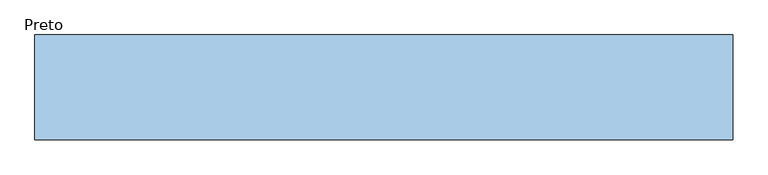
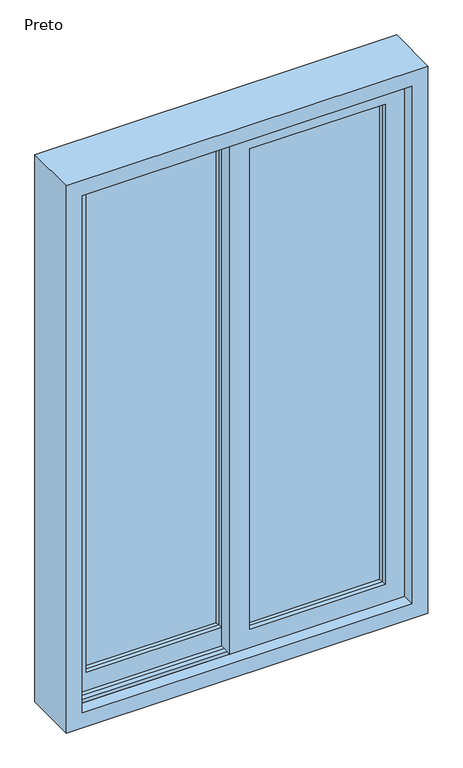
"""IFC4 building model written with IfcOpenShell, lengths in millimetres: window geometry, Blks_Cons Weiku_Janela de Correr 02 Folhas : Preto."""

from ifc_helpers import new_model, si_unit, frame, origin, place, context, project, spatial, polyline, outline, extrude, faceted_brep, source, transform, mapped, element, save


def preto_50c638ee(model_context):
    return source(origin(), model_context, "Body", "SolidModel", [
        faceted_brep([(27.0, -13.0, 898.0), (27.0, -18.0, 898.0), (27.0, -18.0, 2302.0), (27.0, -13.0, 2302.0), (32.0, -18.0, 903.0), (32.0, -18.0, 2297.0), (402.0, -18.0, 2302.0), (402.0, -13.0, 2302.0), (397.0, -18.0, 2297.0), (402.0, -18.0, 898.0), (402.0, -13.0, 898.0), (397.0, -18.0, 903.0)], [[[0, 1, 2, 3]], [[4, 0, 3, 5]], [[3, 2, 6, 7]], [[5, 3, 7, 8]], [[7, 6, 9, 10]], [[8, 7, 10, 11]], [[1, 9, 6, 2], [5, 8, 11, 4]], [[10, 9, 1, 0]], [[11, 10, 0, 4]]]),
        faceted_brep([(402.0, -27.0, 898.0), (402.0, -22.0, 898.0), (402.0, -22.0, 2302.0), (402.0, -27.0, 2302.0), (27.0, -22.0, 2302.0), (27.0, -27.0, 2302.0), (27.0, -22.0, 898.0), (27.0, -27.0, 898.0), (397.0, -22.0, 2297.0), (32.0, -22.0, 2297.0), (32.0, -22.0, 903.0), (397.0, -22.0, 903.0)], [[[0, 1, 2, 3]], [[3, 2, 4, 5]], [[5, 4, 6, 7]], [[1, 6, 4, 2], [8, 9, 10, 11]], [[7, 6, 1, 0]], [[11, 0, 3, 8]], [[8, 3, 5, 9]], [[9, 5, 7, 10]], [[10, 7, 0, 11]]]),
        extrude(outline(polyline([(402.0, -22.0), (27.0, -22.0), (27.0, -18.0), (402.0, -18.0), (402.0, -22.0)])), frame((0.0, 0.0, 898.0), z_axis=(0.0, 0.0, 1.0), x_axis=(1.0, 0.0, 0.0)), (0.0, 0.0, 1.0), 1404.0),
        extrude(outline(polyline([(844.0, 456.0), (2356.0, 456.0), (2356.0, -27.0), (844.0, -27.0), (844.0, 456.0)]), holes=[polyline([(2302.0, 27.0), (2302.0, 402.0), (898.0, 402.0), (898.0, 27.0), (2302.0, 27.0)])]), frame((0.0, -40.0, 0.0), z_axis=(0.0, 1.0, 0.0), x_axis=(0.0, 0.0, 1.0)), (0.0, 0.0, 1.0), 40.0),
        faceted_brep([(-402.0, 27.0, 898.0), (-402.0, 22.0, 898.0), (-402.0, 22.0, 2302.0), (-402.0, 27.0, 2302.0), (-397.0, 22.0, 903.0), (-397.0, 22.0, 2297.0), (-27.0, 22.0, 2302.0), (-27.0, 27.0, 2302.0), (-32.0, 22.0, 2297.0), (-27.0, 22.0, 898.0), (-27.0, 27.0, 898.0), (-32.0, 22.0, 903.0)], [[[0, 1, 2, 3]], [[4, 0, 3, 5]], [[3, 2, 6, 7]], [[5, 3, 7, 8]], [[7, 6, 9, 10]], [[8, 7, 10, 11]], [[1, 9, 6, 2], [5, 8, 11, 4]], [[10, 9, 1, 0]], [[11, 10, 0, 4]]]),
        faceted_brep([(-27.0, 13.0, 898.0), (-27.0, 18.0, 898.0), (-27.0, 18.0, 2302.0), (-27.0, 13.0, 2302.0), (-402.0, 18.0, 2302.0), (-402.0, 13.0, 2302.0), (-402.0, 18.0, 898.0), (-402.0, 13.0, 898.0), (-32.0, 18.0, 2297.0), (-397.0, 18.0, 2297.0), (-397.0, 18.0, 903.0), (-32.0, 18.0, 903.0)], [[[0, 1, 2, 3]], [[3, 2, 4, 5]], [[5, 4, 6, 7]], [[1, 6, 4, 2], [8, 9, 10, 11]], [[7, 6, 1, 0]], [[11, 0, 3, 8]], [[8, 3, 5, 9]], [[9, 5, 7, 10]], [[10, 7, 0, 11]]]),
        extrude(outline(polyline([(-27.0, 18.0), (-402.0, 18.0), (-402.0, 22.0), (-27.0, 22.0), (-27.0, 18.0)])), frame((0.0, 0.0, 898.0), z_axis=(0.0, 0.0, 1.0), x_axis=(1.0, 0.0, 0.0)), (0.0, 0.0, 1.0), 1404.0),
        extrude(outline(polyline([(844.0, 27.0), (2356.0, 27.0), (2356.0, -456.0), (844.0, -456.0), (844.0, 27.0)]), holes=[polyline([(2302.0, -402.0), (2302.0, -27.0), (898.0, -27.0), (898.0, -402.0), (2302.0, -402.0)])]), frame((0.0, 0.0, 0.0), z_axis=(0.0, 1.0, 0.0), x_axis=(0.0, 0.0, 1.0)), (0.0, 0.0, 1.0), 40.0),
        faceted_brep([(456.0, 75.0, 844.0), (-456.0, 75.0, 844.0), (-456.0, 40.0, 844.0), (456.0, 40.0, 844.0), (-456.0, -75.0, 844.0), (456.0, -75.0, 844.0), (456.0, -40.0, 844.0), (-456.0, -40.0, 844.0), (-456.0, -13.0, 844.0), (-456.0, -27.0, 844.0), (456.0, -27.0, 844.0), (456.0, -13.0, 844.0), (-456.0, 27.0, 844.0), (-456.0, 13.0, 844.0), (456.0, 13.0, 844.0), (456.0, 27.0, 844.0), (500.0, 75.0, 800.0), (-500.0, 75.0, 800.0), (-500.0, 75.0, 2400.0), (500.0, 75.0, 2400.0), (456.0, 75.0, 2356.0), (-456.0, 75.0, 2356.0), (-456.0, 40.0, 2356.0), (-456.0, 40.0, 2366.0), (-456.0, 27.0, 2366.0), (-456.0, 27.0, 2356.0), (-456.0, 13.0, 2356.0), (-456.0, 13.0, 2366.0), (-456.0, -13.0, 2366.0), (-456.0, -13.0, 2356.0), (-456.0, -27.0, 2356.0), (-456.0, -27.0, 2366.0), (-456.0, -40.0, 2366.0), (-456.0, -40.0, 2356.0), (-456.0, -75.0, 2356.0), (-456.0, -40.0, 834.0), (-456.0, -27.0, 834.0), (-456.0, -13.0, 834.0), (-456.0, 13.0, 834.0), (-456.0, 27.0, 834.0), (-456.0, 40.0, 834.0), (456.0, 40.0, 834.0), (456.0, 27.0, 834.0), (456.0, 13.0, 834.0), (456.0, -13.0, 834.0), (456.0, -27.0, 834.0), (456.0, -40.0, 834.0), (456.0, -75.0, 2356.0), (456.0, -40.0, 2356.0), (456.0, -40.0, 2366.0), (456.0, -27.0, 2366.0), (456.0, -27.0, 2356.0), (456.0, -13.0, 2356.0), (456.0, -13.0, 2366.0), (456.0, 13.0, 2366.0), (456.0, 13.0, 2356.0), (456.0, 27.0, 2356.0), (456.0, 27.0, 2366.0), (456.0, 40.0, 2366.0), (456.0, 40.0, 2356.0), (-500.0, -75.0, 800.0), (500.0, -75.0, 800.0), (500.0, -75.0, 2400.0), (-500.0, -75.0, 2400.0)], [[[0, 1, 2, 3]], [[4, 5, 6, 7]], [[8, 9, 10, 11]], [[12, 13, 14, 15]], [[16, 17, 18, 19], [1, 0, 20, 21]], [[1, 21, 22, 23, 24, 25, 26, 27, 28, 29, 30, 31, 32, 33, 34, 4, 7, 35, 36, 9, 8, 37, 38, 13, 12, 39, 40, 2]], [[40, 41, 3, 2]], [[20, 0, 3, 41, 42, 15, 14, 43, 44, 11, 10, 45, 46, 6, 5, 47, 48, 49, 50, 51, 52, 53, 54, 55, 56, 57, 58, 59]], [[60, 61, 62, 63], [5, 4, 34, 47]], [[46, 35, 7, 6]], [[45, 10, 9, 36]], [[11, 44, 37, 8]], [[43, 14, 13, 38]], [[15, 42, 39, 12]], [[61, 16, 19, 62]], [[16, 61, 60, 17]], [[17, 60, 63, 18]], [[46, 45, 36, 35]], [[44, 43, 38, 37]], [[42, 41, 40, 39]], [[26, 25, 56, 55]], [[30, 29, 52, 51]], [[21, 20, 59, 22]], [[47, 34, 33, 48]], [[18, 63, 62, 19]], [[55, 54, 27, 26]], [[54, 53, 28, 27]], [[53, 52, 29, 28]], [[51, 50, 31, 30]], [[50, 49, 32, 31]], [[32, 49, 48, 33]], [[58, 23, 22, 59]], [[58, 57, 24, 23]], [[57, 56, 25, 24]]]),
    ])


if __name__ == "__main__":
    model = new_model("IFC4")
    model_context = context("Model", 3, world=origin())
    ifc_project = project(units=[si_unit("LENGTHUNIT", "METRE", prefix="MILLI")], contexts=[model_context])
    site = spatial("IfcSite", under=ifc_project)
    building = spatial("IfcBuilding", under=site)
    placement = place(None, origin())
    preto_shape = preto_50c638ee(model_context)
    element("IfcWindow", 1, ObjectType="Blks_Cons Weiku_Janela de Correr 02 Folhas : Preto", at=placement, inside=building, context=model_context, shape_type="MappedRepresentation", body=[
        mapped(preto_shape, transform((0.0, 0.0, 0.0), x_axis=(1.0, 0.0, 0.0), y_axis=(0.0, 1.0, 0.0), z_axis=(0.0, 0.0, 1.0))),
    ])
    save(model, "model.ifc")

# Revit data of these elements
# Type "Blks_Cons Weiku_Janela de Correr 02 Folhas : Preto"
#   Type Mark = "J26"
#   Type Comments = "Janela de Correr 02 Folhas"
#   Manufacturer = "Weiku"
#   Created By / Criado Por / Creado por = "Blocks"
#   Author URL = "https://BlocksRvt.com/"
#   Author Contact = "info@blocksrvt.com"
#   Assembly Code = "Cons"
#   c [instance default] = 250 mm
#   b [instance default] = 912 mm
#   a [instance default] = 983 mm
#   Rough Width [instance default] = 2000 mm
#   Width [instance default] = 1912 mm
#   Espessura Folha [instance default] = 40 mm
#   Rough Height [instance default] = 1000 mm
#   Height [instance default] = 912 mm
#   Abertura Janela Equerda [instance default] = 0 mm
#   Abertura Janela Direita [instance default] = 0 mm
#   Vidro = .vidro_growarq
#   Vedação = Blks - Rubber - Black
#   Janela = Blks - Plastic - Black - Glazed
#   Wall Closure = (empty or 0)
# Element 1 (IfcWindow, "Blks_Cons Weiku_Janela de Correr 02 Folhas : Preto")
#   c = 200 mm
#   b = 1512 mm
#   a = 483 mm
#   Rough Width = 1000 mm
#   Width = 912 mm
#   Rough Height = 1600 mm
#   Height = 1512 mm
#   Materials on its faces: "Blks - Plastic - Black - Glazed", "Blks - Rubber - Black", ".vidro_growarq"
# Materials
#   ".vidro_growarq": class "Vidro", colour RGB 200 215 215, transparency 0.6, Description = "Vidroverde", Cost = 0
#   "Blks - Rubber - Black": class "Paint/Coating", colour RGB 38 38 38, transparency 0, Cost = 0
#   "Blks - Plastic - Black - Glazed": class "Plastic", colour RGB 25 25 25, transparency 0, Cost = 0
